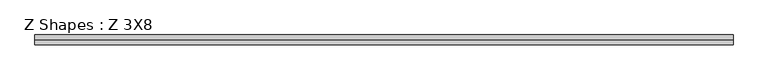
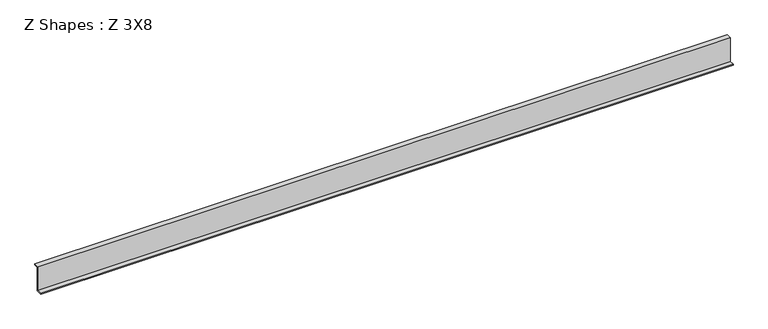
"""IFC4 building model written with IfcOpenShell, lengths in millimetres: beam geometry, Z Shapes : Z 3X8."""

from ifc_helpers import new_model, si_unit, frame, origin, place, context, project, spatial, polyline, outline, extrude, source, transform, mapped, element, save


def z_shapes_z_3x8_f14596aa(model_context):
    return source(origin(), model_context, "Body", "SweptSolid", [
        extrude(outline(polyline([(57.2805719, 92.452825), (27.1991352, 92.452825), (27.1991352, -98.809175), (-18.9194281, -98.809175), (-18.9194281, -92.459175), (19.1805719, -92.459175), (19.1805719, 102.104825), (57.2805719, 102.104825), (57.2805719, 92.452825)])), frame((-2667.0, 0.0, 0.0), z_axis=(1.0, 0.0, 0.0), x_axis=(0.0, 1.0, 0.0)), (0.0, 0.0, 1.0), 5333.9999994),
    ])


if __name__ == "__main__":
    model = new_model("IFC4")
    model_context = context("Model", 3, world=origin())
    ifc_project = project(units=[si_unit("LENGTHUNIT", "METRE", prefix="MILLI")], contexts=[model_context])
    site = spatial("IfcSite", under=ifc_project)
    building = spatial("IfcBuilding", under=site)
    placement = place(None, origin())
    z_shapes_z_3x8_shape = z_shapes_z_3x8_f14596aa(model_context)
    element("IfcBeam", 1, ObjectType="Z Shapes : Z 3X8", at=placement, inside=building, context=model_context, shape_type="MappedRepresentation", body=[
        mapped(z_shapes_z_3x8_shape, transform((0.0, 0.0, 0.0), x_axis=(1.0, 0.0, 0.0), y_axis=(0.0, 1.0, 0.0), z_axis=(0.0, 0.0, 1.0))),
    ])
    save(model, "model.ifc")

# Revit data of these elements
# Type "Z Shapes : Z 3X8"
#   Section Name Key = "W12x26"
#   Assembly Code = "B10"
#   Width = 76.2 mm
#   Web Thickness = 5.842 mm
#   Web Fillet = 7.62 mm
#   Warping Constant = 163001.3 cm⁶
#   Torsional Moment of Inertia = 12.4869 cm⁴
#   Section Area = 7.65 in²
#   Plastic Modulus weak axis = 0.00472801 (stored number, unit not read)
#   Plastic Modulus strong axis = 0.0215278 (stored number, unit not read)
#   Perimeter = 15.0571 m²/m
#   Nominal Weight = 379.441 N/m
#   Moment of Inertia weak axis = 720.08 cm⁴
#   Moment of Inertia strong axis = 8491.12 cm⁴
#   Height = 184.912 mm
#   Flange Thickness = 9.652 mm
#   Elastic Modulus weak axis = 0.00309028 (stored number, unit not read)
#   Elastic Modulus strong axis = 0.0193287 (stored number, unit not read)
#   Centroid Vertical = 92.456 mm
#   Centroid Horizontal = 38.1 mm
#   Length [instance default] = 5' - 0"
#   Structural Material [instance default] = Steel ASTM A992
#   Principal Axes Angle = 0
# Element 1 (IfcBeam, "Z Shapes : Z 3X8")
#   Structural Material = accent 2
#   Materials on its faces: "accent 2"
# Materials
#   "Steel ASTM A992": class "Metal", colour RGB 189 187 185, transparency 0, Description = "Structural steel 50ksi", Cost = 0
#   "accent 2": class "Wood", colour RGB 80 80 80, transparency 0, Description = "Wood framing, thermal airspace", Cost = 0
